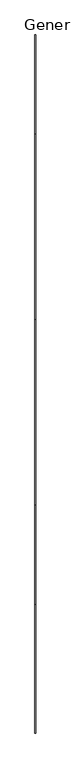
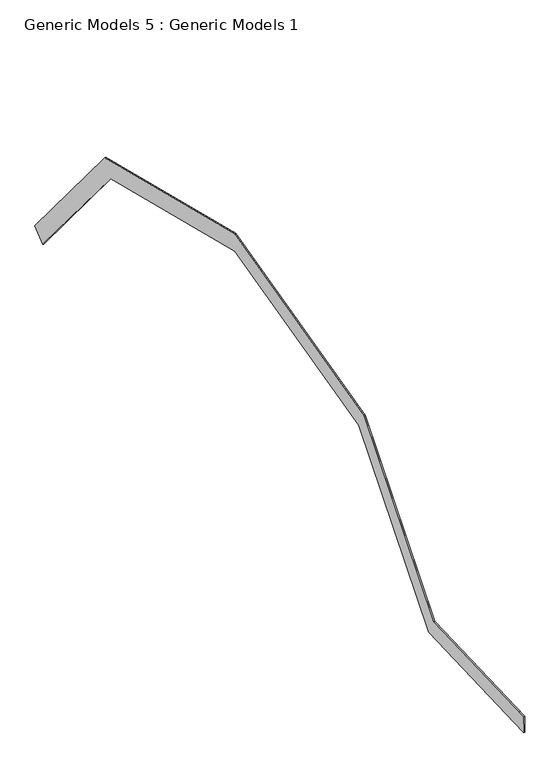
"""IFC4 building model written with IfcOpenShell, lengths in millimetres: proxy geometry, Generic Models 5 : Generic Models 1."""

from ifc_helpers import new_model, si_unit, frame, origin, place, context, project, spatial, polyline, outline, extrude, source, transform, mapped, element, save


def generic_models_5_generic_models_1_9f6939e7(model_context):
    return source(origin(), model_context, "Body", "SweptSolid", [
        extrude(outline(polyline([(11609.9309883, 2984.3405795), (10023.6412719, 4887.8882391), (7113.0570149, 5615.5343034), (4202.4384941, 4887.8796732), (2560.7151338, 2917.8116409), (331.5982071, 2831.1879261), (322.4759913, 3065.9329463), (2434.8673967, 3148.0206952), (4066.3626163, 5105.8149588), (7113.772024, 5867.6673107), (10161.1814316, 5105.8149588), (11797.360301, 3142.4003155), (11609.9309883, 2984.3405795)])), frame((29947.3870052, 0.0, 0.0), z_axis=(1.0, 0.0, 0.0), x_axis=(0.0, 1.0, 0.0)), (0.0, 0.0, 1.0), 13.5023771),
    ])


if __name__ == "__main__":
    model = new_model("IFC4")
    model_context = context("Model", 3, world=origin())
    ifc_project = project(units=[si_unit("LENGTHUNIT", "METRE", prefix="MILLI")], contexts=[model_context])
    site = spatial("IfcSite", under=ifc_project)
    building = spatial("IfcBuilding", under=site)
    placement = place(None, origin())
    generic_models_5_generic_models_1_shape = generic_models_5_generic_models_1_9f6939e7(model_context)
    element("IfcBuildingElementProxy", 1, Name="Generic Models 5 : Generic Models 1", ObjectType="Generic Models 5 : Generic Models 1", at=placement, inside=building, context=model_context, shape_type="MappedRepresentation", body=[
        mapped(generic_models_5_generic_models_1_shape, transform((0.0, 0.0, 0.0), x_axis=(1.0, 0.0, 0.0), y_axis=(0.0, 1.0, 0.0), z_axis=(0.0, 0.0, 1.0))),
    ])
    save(model, "model.ifc")
